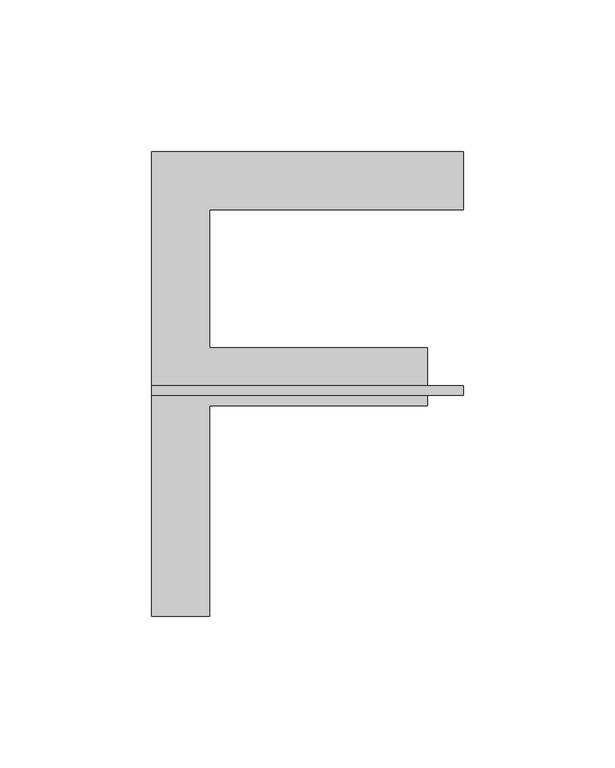
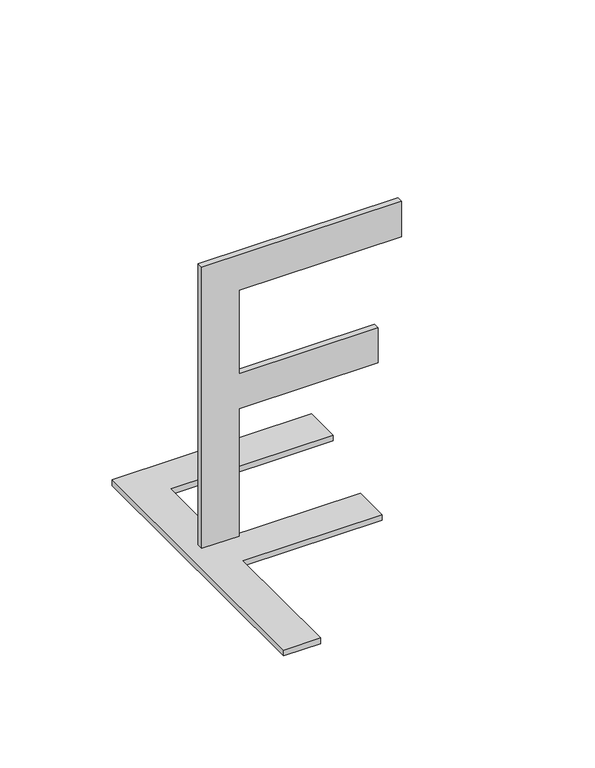
"""IFC4 building model written with IfcOpenShell, lengths in millimetres: proxy geometry, Grid Number1_FedEx : Grid Number1_FedEx."""

from ifc_helpers import new_model, si_unit, frame, origin, origin_with_axes, place, context, project, spatial, polyline, outline, extrude, source, transform, mapped, element, save


def entourage_07adac8a(model_context):
    return source(origin(), model_context, "Body", "SweptSolid", [
        extrude(outline(polyline([(-155.9162444, 146.5840649), (-155.9162444, 299.6794816), (-53.0552614, 299.6794816), (-53.0552614, 280.5425545), (-136.7793174, 280.5425545), (-136.7793174, 235.0923527), (-65.0158408, 235.0923527), (-65.0158408, 215.9554256), (-136.7793174, 215.9554256), (-136.7793174, 146.5840649), (-155.9162444, 146.5840649)])), origin_with_axes(), (0.0, 0.0, 1.0), 3.175),
        extrude(outline(polyline([(14.4798932, -155.9162444), (14.4798932, -136.7793174), (83.8512539, -136.7793174), (83.8512539, -65.0158408), (102.988181, -65.0158408), (102.988181, -136.7793174), (148.4383828, -136.7793174), (148.4383828, -53.0552614), (167.5753099, -53.0552614), (167.5753099, -155.9162444), (14.4798932, -155.9162444)])), frame((0.0, 219.3456765, 0.0), z_axis=(0.0, 1.0, 0.0), x_axis=(0.0, 0.0, 1.0)), (0.0, 0.0, 1.0), 3.175),
    ])


if __name__ == "__main__":
    model = new_model("IFC4")
    model_context = context("Model", 3, world=origin())
    ifc_project = project(units=[si_unit("LENGTHUNIT", "METRE", prefix="MILLI")], contexts=[model_context])
    site = spatial("IfcSite", under=ifc_project)
    building = spatial("IfcBuilding", under=site)
    placement = place(None, origin())
    entourage_shape = entourage_07adac8a(model_context)
    element("IfcBuildingElementProxy", 1, Name="Grid Number1_FedEx : Grid Number1_FedEx", ObjectType="Grid Number1_FedEx : Grid Number1_FedEx", at=placement, inside=building, context=model_context, shape_type="MappedRepresentation", body=[
        mapped(entourage_shape, transform((0.0, 0.0, 0.0), x_axis=(1.0, 0.0, 0.0), y_axis=(0.0, 1.0, 0.0), z_axis=(0.0, 0.0, 1.0))),
    ])
    save(model, "model.ifc")

# Revit data of these elements
# Type "Grid Number1_FedEx : Grid Number1_FedEx"
#   Grid [instance default] = "S.8"
#   Label Width [instance default] = 1' - 0"
#   Half Box Width2 [instance default] = 0' - 6.13846"
#   Half Box Width [instance default] = 0' - 6"
#   Robust [instance default] = yes
#   Height = 0
#   Assembly Code = ""
# Element 1 (IfcBuildingElementProxy, "Grid Number1_FedEx : Grid Number1_FedEx")
#   Grid = "F"
#   Robust = no
#   Materials on its faces: "Letter"
# Materials
#   "Letter": class "Unassigned", colour RGB 178 187 30, transparency 0, Comments = "Rendering appearance not upgraded "
